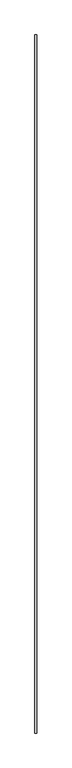
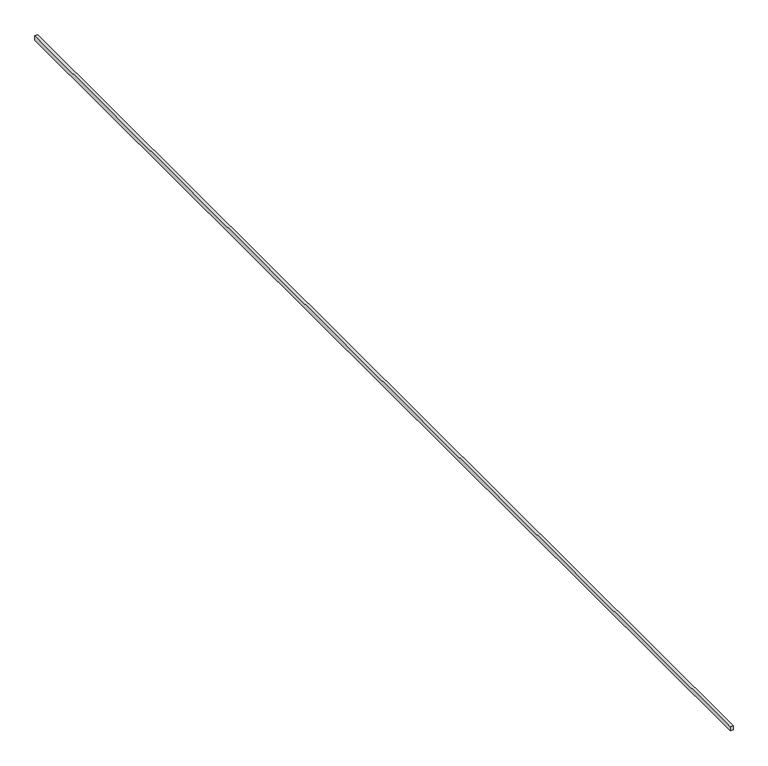
"""IFC4 building model written with IfcOpenShell, lengths in millimetres: proxy geometry, Generic Models 7:Generic Models 1:5:Generic Models 1:5 : Generic Models 7:Generic Models 1:337419:23 : Generic Models 7:Generic Models 1:5:Generic Models 1:5 : Generic Models 7:Generic Models 1:337419:311462."""

from ifc_helpers import new_model, si_unit, frame, origin, place, context, project, spatial, polyline, outline, extrude, source, transform, mapped, element, save


def generic_models_ba025cea(model_context):
    return source(origin(), model_context, "Body", "SweptSolid", [
        extrude(outline(polyline([(578647.3117239, -568215.2163841), (578621.8863239, -568215.2163841), (578621.8863239, -558080.616384), (578647.3117239, -558080.616384), (578647.3117239, -568215.2163841)])), frame((0.0, 0.0, 4876.8), z_axis=(0.0, 0.0, 1.0), x_axis=(1.0, 0.0, 0.0)), (0.0, 0.0, 1.0), 38.6419652),
    ])


if __name__ == "__main__":
    model = new_model("IFC4")
    model_context = context("Model", 3, world=origin())
    ifc_project = project(units=[si_unit("LENGTHUNIT", "METRE", prefix="MILLI")], contexts=[model_context])
    site = spatial("IfcSite", under=ifc_project)
    building = spatial("IfcBuilding", under=site)
    placement = place(None, origin())
    generic_models_shape = generic_models_ba025cea(model_context)
    element("IfcBuildingElementProxy", 1, Name="Generic Models 7:Generic Models 1:5:Generic Models 1:5 : Generic Models 7:Generic Models 1:337419:23 : Generic Models 7:Generic Models 1:5:Generic Models 1:5 : Generic Models 7:Generic Models 1:337419:311462", ObjectType="Generic Models 7:Generic Models 1:5:Generic Models 1:5 : Generic Models 7:Generic Models 1:337419:23 : Generic Models 7:Generic Models 1:5:Generic Models 1:5 : Generic Models 7:Generic Models 1:337419:311462", at=placement, inside=building, context=model_context, shape_type="MappedRepresentation", body=[
        mapped(generic_models_shape, transform((0.0, 0.0, 0.0), x_axis=(1.0, 0.0, 0.0), y_axis=(0.0, 1.0, 0.0), z_axis=(0.0, 0.0, 1.0))),
    ])
    save(model, "model.ifc")

# Revit data of these elements
# Type "Generic Models 7:Generic Models 1:5:Generic Models 1:5 : Generic Models 7:Generic Models 1:337419:23 : Generic Models 7:Generic Models 1:5:Generic Models 1:5 : Generic Models 7:Generic Models 1:337419:311462"
#   NameOverride = "Generic Models 7:Generic Models 1:5:Generic Models 1:5 : Generic Models 7:Generic Models 1:337419:311462"
#   ObjectTypeOverride = "Generic Models 1:5 : Generic Models 7:Generic Models 1:337419"
#   Reference = "Generic Models 1"
#   Tag = "311462"
# Element 1 (IfcBuildingElementProxy, "Generic Models 7:Generic Models 1:5:Generic Models 1:5 : Generic Models 7:Generic Models 1:337419:23 : Generic Models 7:Generic Models 1:5:Generic Models 1:5 : Generic Models 7:Generic Models 1:337419:311462")
#   Materials on its faces: "RIGID INSULATION AT GIRTS/JAMB - (CLASS A FLAME SPREAD)"
# Materials
#   "RIGID INSULATION AT GIRTS/JAMB - (CLASS A FLAME SPREAD)": class "Unassigned", colour RGB 205 188 106, transparency 0, Cost = 0
